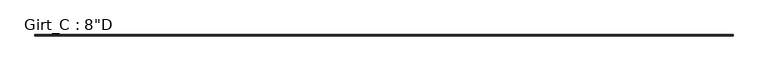
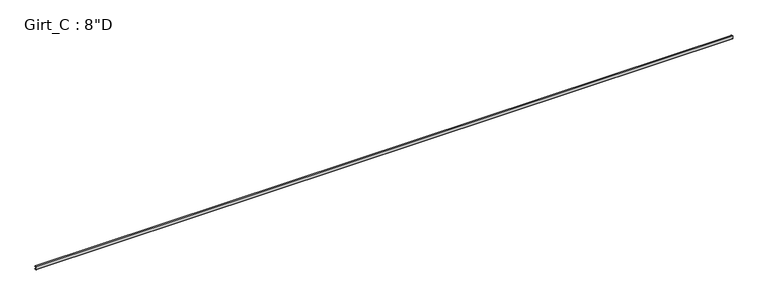
"""IFC4 building model written with IfcOpenShell, lengths in millimetres: beam geometry."""

from ifc_helpers import new_model, si_unit, point, frame, frame_2d, origin, place, context, project, spatial, polyline, circle_curve, trimmed, segment, composite_curve, outline, extrude, source, transform, mapped, element, save


def beam_eb43aaad(model_context):
    return source(origin(), model_context, "Body", "SweptSolid", [
        extrude(outline(composite_curve([segment(polyline([(63.5, 101.6), (75.745104, 87.0068534), (73.6169367, 85.221109), (62.204539, 98.821875), (3.3005807, 98.821875)]), True, "CONTINUOUS"), segment(trimmed(circle_curve(frame_2d((3.3741066, 96.8381931)), 1.9850441), [point((3.3005807, 98.821875))], [point((1.3890625, 96.8381931))], True, "CARTESIAN"), True, "CONTINUOUS"), segment(polyline([(1.3890625, 96.8381931), (1.3890625, -96.8389339)]), True, "CONTINUOUS"), segment(trimmed(circle_curve(frame_2d((3.3748024, -96.8389339)), 1.9857399), [point((1.3890625, -96.8389339))], [point((3.2694106, -98.821875))], True, "CARTESIAN"), True, "CONTINUOUS"), segment(polyline([(3.2694106, -98.821875), (62.204539, -98.821875), (73.6169367, -85.221109), (75.745104, -87.0068534), (63.5, -101.6), (3.3734375, -101.6)]), True, "CONTINUOUS"), segment(trimmed(circle_curve(frame_2d((3.3734375, -96.8375)), 4.7625), [point((3.3734375, -101.6))], [point((-1.3890625, -96.8375))], False, "CARTESIAN"), True, "CONTINUOUS"), segment(polyline([(-1.3890625, -96.8375), (-1.3890625, 96.8375)]), True, "CONTINUOUS"), segment(trimmed(circle_curve(frame_2d((3.3734375, 96.8375)), 4.7625), [point((-1.3890625, 96.8375))], [point((3.3734375, 101.6))], False, "CARTESIAN"), True, "CONTINUOUS"), segment(polyline([(3.3734375, 101.6), (63.5, 101.6)]), True, "CONTINUOUS")], self_intersect=False)), frame((-19951.7, 0.0, 0.0), z_axis=(1.0, 0.0, 0.0), x_axis=(0.0, 1.0, 0.0)), (0.0, 0.0, 1.0), 39973.6818),
    ])


if __name__ == "__main__":
    model = new_model("IFC4")
    model_context = context("Model", 3, world=origin())
    ifc_project = project(units=[si_unit("LENGTHUNIT", "METRE", prefix="MILLI")], contexts=[model_context])
    site = spatial("IfcSite", under=ifc_project)
    building = spatial("IfcBuilding", under=site)
    placement = place(None, origin())
    beam_shape = beam_eb43aaad(model_context)
    element("IfcBeam", 1, ObjectType="Girt_C : 8\"D", at=placement, inside=building, context=model_context, shape_type="MappedRepresentation", body=[
        mapped(beam_shape, transform((0.0, 0.0, 0.0), x_axis=(1.0, 0.0, 0.0), y_axis=(0.0, 1.0, 0.0), z_axis=(0.0, 0.0, 1.0))),
    ])
    save(model, "model.ifc")

# Revit data of these elements
# Type "Girt_C : 8\"D"
#   Web_Thickness = 0' - 0 7/64"
#   Length [instance default] = 10' - 0"
#   Leg_1 = 0' - 2 1/2"
#   Height = 0' - 8"
#   Structural Material [instance default] = none
# Element 1 (IfcBeam, "Girt_C : 8\"D")
#   Structural Material = Steel
#   Materials on its faces: "Steel"
# Materials
#   "Steel": class "Metal", colour RGB 118 118 114, transparency 0, Description = "Steel, mill finish", Cost = 0
